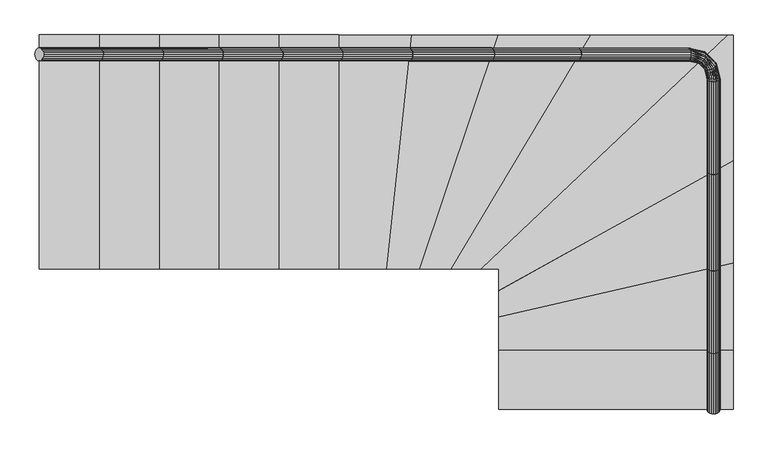
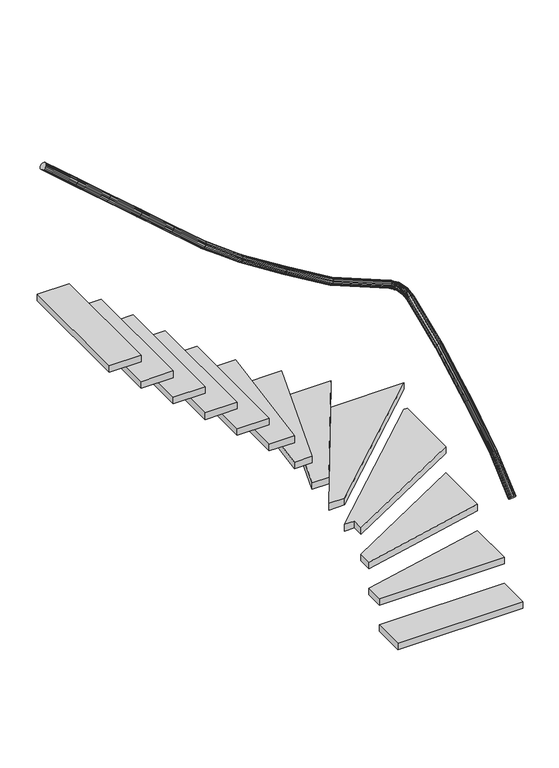
"""IFC4 building model written with IfcOpenShell, lengths in millimetres: stair geometry, 0_3d."""

import ifcopenshell
import ifcopenshell.guid

model = None  # the IFC model being written
_history = None  # IfcOwnerHistory: only IFC2X3 demands one
_inside = {}  # id of a spatial element -> (the spatial element, [elements in it])
_under = {}  # id of a project, library or spatial element -> (it, [spatial elements below it])
_declared = {}  # id of a project -> (the project, [libraries it declares])
_typed = {}  # id of a type object -> (the type object, [elements of that type])
_made_of = {}  # id of a material, layer set ... -> (it, [elements and type objects made of it])


def new_model(schema):
    """Start an empty IFC model of exactly this schema.

    Asked for "IFC4X3", IfcOpenShell would pick the latest addendum, in which some entities
    have other attributes; the version numbers below select the first issue.
    IFC2X3 requires an IfcOwnerHistory on every rooted entity: one is made here for all.
    """
    global model, _history
    if schema == "IFC4X3":
        model = ifcopenshell.file(schema_version=(4, 3, 0, 0))
    else:
        model = ifcopenshell.file(schema=schema)
    _inside.clear()
    _under.clear()
    _declared.clear()
    _typed.clear()
    _made_of.clear()
    _history = None
    if model.schema == "IFC2X3":
        org = make("IfcOrganization", Name="unknown")
        user = make(
            "IfcPersonAndOrganization",
            ThePerson=make("IfcPerson", FamilyName="unknown"),
            TheOrganization=org,
        )
        app = make(
            "IfcApplication",
            ApplicationDeveloper=org,
            Version="unknown",
            ApplicationFullName="unknown",
            ApplicationIdentifier="unknown",
        )
        _history = make(
            "IfcOwnerHistory",
            OwningUser=user,
            OwningApplication=app,
            ChangeAction="ADDED",
            CreationDate=0,
        )
    return model


def make(cls, **values):
    """One entity of the class cls with the attributes given. An attribute that is None is left unset."""
    return model.create_entity(
        cls, **{name: value for name, value in values.items() if value is not None}
    )


def rooted(cls, **values):
    """An entity with a GlobalId (a new one), such as an element, a storey or a relation."""
    return make(cls, GlobalId=ifcopenshell.guid.new(), OwnerHistory=_history, **values)


def si_unit(unit_type, name, prefix=None):
    """IfcSIUnit, for example si_unit("LENGTHUNIT", "METRE", prefix="MILLI")."""
    return make("IfcSIUnit", UnitType=unit_type, Prefix=prefix, Name=name)


def assignment(units):
    """IfcUnitAssignment: the units of a project."""
    return None if units is None else make("IfcUnitAssignment", Units=units)


def point(xyz):
    """IfcCartesianPoint."""
    return None if xyz is None else make("IfcCartesianPoint", Coordinates=xyz)


def direction(xyz):
    """IfcDirection."""
    return None if xyz is None else make("IfcDirection", DirectionRatios=xyz)


def frame(location, z_axis=None, x_axis=None):
    """IfcAxis2Placement3D, a coordinate frame: its origin and axes. An axis left out is left unset."""
    return make(
        "IfcAxis2Placement3D",
        Location=point(location),
        Axis=direction(z_axis),
        RefDirection=direction(x_axis),
    )


def origin():
    """The frame at (0, 0, 0) with its axes left unset."""
    return frame((0.0, 0.0, 0.0))


def origin_with_axes():
    """The frame at (0, 0, 0) with the z axis (0, 0, 1) and the x axis (1, 0, 0) written out."""
    return frame((0.0, 0.0, 0.0), z_axis=(0.0, 0.0, 1.0), x_axis=(1.0, 0.0, 0.0))


def place(relative_to, where):
    """IfcLocalPlacement: puts the frame where relative to a parent placement (None: the world)."""
    return make(
        "IfcLocalPlacement", PlacementRelTo=relative_to, RelativePlacement=where
    )


def context(
    kind, dimensions, precision=None, world=None, true_north=None, identifier=None
):
    """IfcGeometricRepresentationContext, for example the 3D "Model" context."""
    return make(
        "IfcGeometricRepresentationContext",
        ContextIdentifier=identifier,
        ContextType=kind,
        CoordinateSpaceDimension=dimensions,
        Precision=precision,
        WorldCoordinateSystem=world,
        TrueNorth=true_north,
    )


def project(units=None, contexts=None):
    """IfcProject with its units and contexts."""
    return rooted(
        "IfcProject",
        Name="project",
        RepresentationContexts=contexts,
        UnitsInContext=assignment(units),
    )


def spatial(cls, under=None, at=None, **own):
    """A site, building, storey or space (cls), placed at a placement, below another one or the project."""
    s = rooted(cls, ObjectPlacement=at, **own)
    if under is not None:
        _under.setdefault(under.id(), (under, []))[1].append(s)
    return s


def polyline(points):
    """IfcPolyline through the points."""
    return make("IfcPolyline", Points=[point(p) for p in points])


def outline(outer, holes=None, kind="AREA"):
    """IfcArbitraryClosedProfileDef: a profile drawn as a closed curve; with holes, ...WithVoids."""
    if holes is None:
        return make("IfcArbitraryClosedProfileDef", ProfileType=kind, OuterCurve=outer)
    return make(
        "IfcArbitraryProfileDefWithVoids",
        ProfileType=kind,
        OuterCurve=outer,
        InnerCurves=holes,
    )


def extrude(swept, where, along, depth):
    """IfcExtrudedAreaSolid: the profile swept, set in the frame where, extruded along a direction by depth."""
    return make(
        "IfcExtrudedAreaSolid",
        SweptArea=swept,
        Position=where,
        ExtrudedDirection=direction(along),
        Depth=depth,
    )


def faces_of(points, faces, orient=None, outer=None):
    """IfcFace entities. A face is a list of loops; a loop is a list of indices into points, from 0.

    orient and outer hold one flag for each loop. By default every Orientation is true, the
    first loop of a face is its IfcFaceOuterBound and the others are IfcFaceBound.
    """
    made = []
    for i, loops in enumerate(faces):
        bounds = []
        for j, loop in enumerate(loops):
            is_outer = j == 0 if outer is None else outer[i][j]
            bounds.append(
                make(
                    "IfcFaceOuterBound" if is_outer else "IfcFaceBound",
                    Bound=make("IfcPolyLoop", Polygon=[points[k] for k in loop]),
                    Orientation=True if orient is None else orient[i][j],
                )
            )
        made.append(make("IfcFace", Bounds=bounds))
    return made


def faceted_brep(points, faces, orient=None, outer=None, voids=None):
    """IfcFacetedBrep: a solid bounded by flat faces; with voids (closed shells), ...WithVoids."""
    shared = [point(p) for p in points]
    hull = make("IfcClosedShell", CfsFaces=faces_of(shared, faces, orient, outer))
    if voids is None:
        return make("IfcFacetedBrep", Outer=hull)
    return make(
        "IfcFacetedBrepWithVoids",
        Outer=hull,
        Voids=[
            make(cls, CfsFaces=faces_of(shared, fs, o, b)) for cls, fs, o, b in voids
        ],
    )


def shape(context_of_items, identifier, shape_type, items):
    """IfcShapeRepresentation: the items that make up one representation, for example the "Body"."""
    return make(
        "IfcShapeRepresentation",
        ContextOfItems=context_of_items,
        RepresentationIdentifier=identifier,
        RepresentationType=shape_type,
        Items=items,
    )


def source(mapping_origin, context_of_items, identifier, shape_type, items):
    """IfcRepresentationMap: a shape defined once, which mapped items show again and again."""
    return make(
        "IfcRepresentationMap",
        MappingOrigin=mapping_origin,
        MappedRepresentation=shape(context_of_items, identifier, shape_type, items),
    )


def transform(
    local_origin,
    x_axis=None,
    y_axis=None,
    z_axis=None,
    scale=None,
    scale2=None,
    scale3=None,
    uniform=True,
):
    """IfcCartesianTransformationOperator3D, or its non-uniform kind. x_axis, y_axis, z_axis: its Axis1, 2, 3."""
    if uniform:
        return make(
            "IfcCartesianTransformationOperator3D",
            Axis1=direction(x_axis),
            Axis2=direction(y_axis),
            LocalOrigin=point(local_origin),
            Scale=scale,
            Axis3=direction(z_axis),
        )
    return make(
        "IfcCartesianTransformationOperator3DnonUniform",
        Axis1=direction(x_axis),
        Axis2=direction(y_axis),
        LocalOrigin=point(local_origin),
        Scale=scale,
        Axis3=direction(z_axis),
        Scale2=scale2,
        Scale3=scale3,
    )


def mapped(mapping_source, mapping_target):
    """IfcMappedItem: shows the shape of a source again, moved by a transform."""
    return make(
        "IfcMappedItem", MappingSource=mapping_source, MappingTarget=mapping_target
    )


def made_of(thing, what):
    """Note that an element or type object is made of a material, layer set ...; save() writes the relation."""
    if what is not None:
        _made_of.setdefault(what.id(), (what, []))[1].append(thing)
    return thing


def element(
    cls,
    number,
    at=None,
    inside=None,
    cuts=None,
    type_object=None,
    material=None,
    context=None,
    identifier="Body",
    shape_type=None,
    held_by="IfcProductDefinitionShape",
    body=None,
    shapes=None,
    **own,
):
    """One element of the class cls, such as IfcWall. Its Tag is "e" and its number.

    at: its placement. inside: the storey or other place that contains it. cuts: it is an
    opening in that element (IfcRelVoidsElement). A single representation is given by context,
    identifier, shape_type and body (its items); several are given by shapes. held_by: the class
    of the entity that holds the representations. save() writes the other relations.
    """
    e = rooted(cls, Tag="e%d" % number, ObjectPlacement=at, **own)
    if body is not None:
        shapes = [shape(context, identifier, shape_type, body)]
    if shapes is not None:
        e.Representation = make(held_by, Representations=shapes)
    if inside is not None:
        _inside.setdefault(inside.id(), (inside, []))[1].append(e)
    if cuts is not None:
        rooted(
            "IfcRelVoidsElement", RelatingBuildingElement=cuts, RelatedOpeningElement=e
        )
    if type_object is not None:
        _typed.setdefault(type_object.id(), (type_object, []))[1].append(e)
    return made_of(e, material)


def aggregate(whole, parts):
    """IfcRelAggregates: a whole, such as a stair, and the parts it consists of."""
    return rooted("IfcRelAggregates", RelatingObject=whole, RelatedObjects=parts)


def save(model, path):
    """Write the relations noted so far, then the file.

    IfcRelAggregates (storeys below a building ...), IfcRelContainedInSpatialStructure (elements
    in a storey), IfcRelDefinesByType, IfcRelAssociatesMaterial and IfcRelDeclares: one each for
    every whole, place, type object, material and project.
    """
    for whole, parts in _under.values():
        aggregate(whole, parts)
    for where, things in _inside.values():
        rooted(
            "IfcRelContainedInSpatialStructure",
            RelatedElements=things,
            RelatingStructure=where,
        )
    for kind, things in _typed.values():
        rooted("IfcRelDefinesByType", RelatedObjects=things, RelatingType=kind)
    for what, things in _made_of.values():
        rooted("IfcRelAssociatesMaterial", RelatedObjects=things, RelatingMaterial=what)
    for by, libraries in _declared.values():
        rooted("IfcRelDeclares", RelatingContext=by, RelatedDefinitions=libraries)
    model.write(path)


def stair_d2e62eaa(model_context):
    return source(origin(), model_context, "Body", "SolidModel", [
        extrude(outline(polyline([(1597.2416565, 556.9712063), (1477.0914164, 556.9712063), (1776.8509962, 1456.9712063), (2132.6926944, 1456.9712063), (1597.2416565, 556.9712063)])), frame((0.0, 0.0, 1000.0), z_axis=(0.0, 0.0, 1.0), x_axis=(1.0, 0.0, 0.0)), (0.0, 0.0, 1.0), 50.0),
        extrude(outline(polyline([(1781.5730429, 246.9712063), (1781.5730429, 374.004016), (2681.5730429, 579.9383967), (2681.5730429, 246.9712063), (1781.5730429, 246.9712063)])), frame((0.0, 0.0, 200.0), z_axis=(0.0, 0.0, 1.0), x_axis=(1.0, 0.0, 0.0)), (0.0, 0.0, 1.0), 50.0),
        faceted_brep([(1747.6858023, 1405.7476192, 2062.7493649), (1751.8710312, 1406.9712063, 2069.5592366), (1756.0562602, 1405.7476192, 2076.3691083), (1759.8318097, 1402.1966312, 2082.5123824), (1762.8281028, 1396.6658376, 2087.3877122), (1764.7518414, 1389.6966312, 2090.5178667), (1765.4147166, 1381.9712063, 2091.5964444), (1764.7518414, 1374.2457815, 2090.5178667), (1762.8281028, 1367.276575, 2087.3877122), (1759.8318097, 1361.7457815, 2082.5123824), (1756.0562602, 1358.1947934, 2076.3691083), (1751.8710312, 1356.9712063, 2069.5592366), (1747.6858023, 1358.1947934, 2062.7493649), (1743.9102527, 1361.7457815, 2056.6060909), (1740.9139596, 1367.276575, 2051.730761), (1738.9902211, 1374.2457815, 2048.6006065), (1738.3273459, 1381.9712063, 2047.5220288), (1738.9902211, 1389.6966312, 2048.6006065), (1740.9139596, 1396.6658376, 2051.730761), (1743.9102527, 1402.1966312, 2056.6060909), (1441.2565059, 1405.7476192, 2276.1520608), (1436.7292732, 1406.9712063, 2269.5592366), (1432.2020405, 1405.7476192, 2262.9664125), (1428.1179649, 1402.1966312, 2257.0189399), (1424.8768241, 1396.6658376, 2252.2989989), (1422.7958836, 1389.6966312, 2249.2686103), (1422.0788404, 1381.9712063, 2248.2244095), (1422.7958836, 1374.2457815, 2249.2686103), (1424.8768241, 1367.276575, 2252.2989989), (1428.1179649, 1361.7457815, 2257.0189399), (1432.2020405, 1358.1947934, 2262.9664125), (1436.7292732, 1356.9712063, 2269.5592366), (1441.2565059, 1358.1947934, 2276.1520608), (1445.3405815, 1361.7457815, 2282.0995333), (1448.5817223, 1367.276575, 2286.8194743), (1450.6626628, 1374.2457815, 2289.8498629), (1451.379706, 1381.9712063, 2290.8940637), (1450.6626628, 1389.6966312, 2289.8498629), (1448.5817223, 1396.6658376, 2286.8194743), (1445.3405815, 1402.1966312, 2282.0995333)], [[[0, 1, 2, 3, 4, 5, 6, 7, 8, 9, 10, 11, 12, 13, 14, 15, 16, 17, 18, 19]], [[20, 21, 22, 23, 24, 25, 26, 27, 28, 29, 30, 31, 32, 33, 34, 35, 36, 37, 38, 39]], [[2, 1, 21, 20]], [[3, 2, 20, 39]], [[4, 3, 39, 38]], [[5, 4, 38, 37]], [[6, 5, 37, 36]], [[7, 6, 36, 35]], [[8, 7, 35, 34]], [[9, 8, 34, 33]], [[10, 9, 33, 32]], [[11, 10, 32, 31]], [[12, 11, 31, 30]], [[13, 12, 30, 29]], [[14, 13, 29, 28]], [[15, 14, 28, 27]], [[16, 15, 27, 26]], [[17, 16, 26, 25]], [[18, 17, 25, 24]], [[19, 18, 24, 23]], [[0, 19, 23, 22]], [[1, 0, 22, 21]]]),
        extrude(outline(polyline([(1711.5730429, 556.9712063), (1597.2416565, 556.9712063), (2132.6926944, 1456.9712063), (2658.9026268, 1456.9712063), (1711.5730429, 556.9712063)])), frame((0.0, 0.0, 800.0), z_axis=(0.0, 0.0, 1.0), x_axis=(1.0, 0.0, 0.0)), (0.0, 0.0, 1.0), 50.0),
        extrude(outline(polyline([(476.9712063, 556.9712063), (246.9712063, 556.9712063), (246.9712063, 1456.9712063), (476.9712063, 1456.9712063), (476.9712063, 556.9712063)])), frame((0.0, 0.0, 2200.0), z_axis=(0.0, 0.0, 1.0), x_axis=(1.0, 0.0, 0.0)), (0.0, 0.0, 1.0), 50.0),
        faceted_brep([(2630.3494558, 1289.6562562, 1611.0200809), (2631.5730429, 1286.5654708, 1618.3905793), (2630.3494558, 1283.4746854, 1625.7610778), (2626.7984678, 1280.6864477, 1632.4101004), (2621.2676742, 1278.4736897, 1637.6867947), (2614.2984678, 1277.0530116, 1641.074641), (2606.5730429, 1276.5634793, 1642.2420132), (2598.8476181, 1277.0530116, 1641.074641), (2591.8784116, 1278.4736897, 1637.6867947), (2586.3476181, 1280.6864477, 1632.4101004), (2582.79663, 1283.4746854, 1625.7610778), (2581.5730429, 1286.5654708, 1618.3905793), (2582.79663, 1289.6562562, 1611.0200809), (2586.3476181, 1292.4444939, 1604.3710583), (2591.8784116, 1294.6572519, 1599.094364), (2598.8476181, 1296.07793, 1595.7065177), (2606.5730429, 1296.5674623, 1594.5391455), (2614.2984678, 1296.07793, 1595.7065177), (2621.2676742, 1294.6572519, 1599.094364), (2626.7984678, 1292.4444939, 1604.3710583), (2616.5930378, 1348.981721, 1644.4666407), (2617.4087642, 1344.9399789, 1651.4217307), (2615.9975628, 1340.119684, 1657.6960081), (2612.4975719, 1334.9926804, 1662.6753028), (2607.2513949, 1330.060835, 1665.8722068), (2600.7725643, 1325.8069111, 1666.9737849), (2593.6952731, 1322.6473125, 1665.8722068), (2586.7122958, 1320.8913226, 1662.6753028), (2580.507175, 1320.71083, 1657.6960081), (2575.6873111, 1322.1235026, 1651.4217307), (2572.7245059, 1324.9910581, 1644.4666407), (2571.9087795, 1329.0328002, 1637.5115507), (2573.3199809, 1333.8530951, 1631.2372733), (2576.8199719, 1338.9800987, 1626.2579786), (2582.0661488, 1343.9119441, 1623.0610746), (2588.5449795, 1348.165868, 1621.9594966), (2595.6222707, 1351.3254666, 1623.0610746), (2602.605248, 1353.0814565, 1626.2579786), (2608.8103688, 1353.2619491, 1631.2372733), (2613.6302327, 1351.8492765, 1637.5115507), (2573.4194125, 1392.0411015, 1672.0001373), (2576.2683384, 1389.0986856, 1678.9715199), (2577.6691227, 1384.2945329, 1685.260495), (2577.4846471, 1378.0989073, 1690.251454), (2575.7329691, 1371.11828, 1693.4558469), (2572.5855554, 1364.0359633, 1694.5600054), (2568.3504965, 1357.5452238, 1693.4558469), (2563.4423498, 1352.2814202, 1690.251454), (2558.3415586, 1348.7598103, 1685.260495), (2553.547424, 1347.3251138, 1678.9715199), (2549.5292294, 1348.1177689, 1672.0001373), (2546.6803035, 1351.0601849, 1665.0287546), (2545.2795191, 1355.8643376, 1658.7397795), (2545.4639948, 1362.0599631, 1653.7488206), (2547.2156727, 1369.0405904, 1650.5444277), (2550.3630865, 1376.1229071, 1649.4402691), (2554.5981453, 1382.6136466, 1650.5444277), (2559.5062921, 1387.8774503, 1653.7488206), (2564.6070832, 1391.3990601, 1658.7397795), (2569.4012178, 1392.8337566, 1665.0287546), (2510.8572333, 1406.9712063, 1697.6556493), (2513.867569, 1405.7476192, 1705.05937), (2516.583232, 1402.1966312, 1711.7383629), (2518.7383944, 1396.6658376, 1717.0388417), (2520.1220939, 1389.6966312, 1720.4419586), (2520.5988842, 1381.9712063, 1721.6145928), (2520.1220939, 1374.2457815, 1720.4419586), (2518.7383944, 1367.276575, 1717.0388417), (2516.583232, 1361.7457815, 1711.7383629), (2513.867569, 1358.1947934, 1705.05937), (2510.8572333, 1356.9712063, 1697.6556493), (2507.8468977, 1358.1947934, 1690.2519286), (2505.1312346, 1361.7457815, 1683.5729357), (2502.9760722, 1367.276575, 1678.2724569), (2501.5923728, 1374.2457815, 1674.86934), (2501.1155825, 1381.9712063, 1673.6967059), (2501.5923728, 1389.6966312, 1674.86934), (2502.9760722, 1396.6658376, 1678.2724569), (2505.1312346, 1402.1966312, 1683.5729357), (2507.8468977, 1405.7476192, 1690.2519286), (2091.6401721, 1405.7476192, 1876.7360506), (2088.0717746, 1406.9712063, 1869.5592366), (2084.503377, 1405.7476192, 1862.3824226), (2081.2842791, 1402.1966312, 1855.9081251), (2078.7295885, 1396.6658376, 1850.7700936), (2077.0893762, 1389.6966312, 1847.4712742), (2076.5241975, 1381.9712063, 1846.3345786), (2077.0893762, 1374.2457815, 1847.4712742), (2078.7295885, 1367.276575, 1850.7700936), (2081.2842791, 1361.7457815, 1855.9081251), (2084.503377, 1358.1947934, 1862.3824226), (2088.0717746, 1356.9712063, 1869.5592366), (2091.6401721, 1358.1947934, 1876.7360506), (2094.8592701, 1361.7457815, 1883.2103481), (2097.4139607, 1367.276575, 1888.3483797), (2099.054173, 1374.2457815, 1891.647199), (2099.6193516, 1381.9712063, 1892.7838947), (2099.054173, 1389.6966312, 1891.647199), (2097.4139607, 1396.6658376, 1888.3483797), (2094.8592701, 1402.1966312, 1883.2103481)], [[[0, 1, 2, 3, 4, 5, 6, 7, 8, 9, 10, 11, 12, 13, 14, 15, 16, 17, 18, 19]], [[2, 1, 20]], [[21, 2, 20]], [[3, 2, 21]], [[22, 3, 21]], [[4, 3, 22]], [[23, 4, 22]], [[5, 4, 23]], [[24, 5, 23]], [[6, 5, 24]], [[25, 6, 24]], [[7, 6, 25]], [[26, 7, 25]], [[8, 7, 26]], [[27, 8, 26]], [[9, 8, 27]], [[28, 9, 27]], [[10, 9, 28]], [[29, 10, 28]], [[11, 10, 29]], [[30, 11, 29]], [[12, 11, 30]], [[31, 12, 30]], [[13, 12, 31]], [[32, 13, 31]], [[14, 13, 32]], [[33, 14, 32]], [[15, 14, 33]], [[34, 15, 33]], [[16, 15, 34]], [[35, 16, 34]], [[17, 16, 35]], [[36, 17, 35]], [[18, 17, 36]], [[37, 18, 36]], [[19, 18, 37]], [[38, 19, 37]], [[0, 19, 38]], [[39, 0, 38]], [[1, 0, 39]], [[20, 1, 39]], [[21, 20, 40]], [[41, 21, 40]], [[22, 21, 41]], [[42, 22, 41]], [[23, 22, 42]], [[43, 23, 42]], [[24, 23, 43]], [[44, 24, 43]], [[25, 24, 44]], [[45, 25, 44]], [[26, 25, 45]], [[46, 26, 45]], [[27, 26, 46]], [[47, 27, 46]], [[28, 27, 47]], [[48, 28, 47]], [[29, 28, 48]], [[49, 29, 48]], [[30, 29, 49]], [[50, 30, 49]], [[31, 30, 50]], [[51, 31, 50]], [[32, 31, 51]], [[52, 32, 51]], [[33, 32, 52]], [[53, 33, 52]], [[34, 33, 53]], [[54, 34, 53]], [[35, 34, 54]], [[55, 35, 54]], [[36, 35, 55]], [[56, 36, 55]], [[37, 36, 56]], [[57, 37, 56]], [[38, 37, 57]], [[58, 38, 57]], [[39, 38, 58]], [[59, 39, 58]], [[20, 39, 59]], [[40, 20, 59]], [[41, 40, 60]], [[61, 41, 60]], [[42, 41, 61]], [[62, 42, 61]], [[43, 42, 62]], [[63, 43, 62]], [[44, 43, 63]], [[64, 44, 63]], [[45, 44, 64]], [[65, 45, 64]], [[46, 45, 65]], [[66, 46, 65]], [[47, 46, 66]], [[67, 47, 66]], [[48, 47, 67]], [[68, 48, 67]], [[49, 48, 68]], [[69, 49, 68]], [[50, 49, 69]], [[70, 50, 69]], [[51, 50, 70]], [[71, 51, 70]], [[52, 51, 71]], [[72, 52, 71]], [[53, 52, 72]], [[73, 53, 72]], [[54, 53, 73]], [[74, 54, 73]], [[55, 54, 74]], [[75, 55, 74]], [[56, 55, 75]], [[76, 56, 75]], [[57, 56, 76]], [[77, 57, 76]], [[58, 57, 77]], [[78, 58, 77]], [[59, 58, 78]], [[79, 59, 78]], [[40, 59, 79]], [[60, 40, 79]], [[80, 81, 82, 83, 84, 85, 86, 87, 88, 89, 90, 91, 92, 93, 94, 95, 96, 97, 98, 99]], [[61, 60, 81, 80]], [[62, 61, 80, 99]], [[63, 62, 99, 98]], [[64, 63, 98, 97]], [[65, 64, 97, 96]], [[66, 65, 96, 95]], [[67, 66, 95, 94]], [[68, 67, 94, 93]], [[69, 68, 93, 92]], [[70, 69, 92, 91]], [[71, 70, 91, 90]], [[72, 71, 90, 89]], [[73, 72, 89, 88]], [[74, 73, 88, 87]], [[75, 74, 87, 86]], [[76, 75, 86, 85]], [[77, 76, 85, 84]], [[78, 77, 84, 83]], [[79, 78, 83, 82]], [[60, 79, 82, 81]]]),
        faceted_brep([(2630.3494558, 935.1107738, 1462.3430272), (2631.5730429, 931.6520604, 1469.5592366), (2630.3494558, 928.193347, 1476.775446), (2626.7984678, 925.0731965, 1483.2852826), (2621.2676742, 922.5970311, 1488.4515182), (2614.2984678, 921.0072351, 1491.7684456), (2606.5730429, 920.4594287, 1492.9113809), (2598.8476181, 921.0072351, 1491.7684456), (2591.8784116, 922.5970311, 1488.4515182), (2586.3476181, 925.0731965, 1483.2852826), (2582.79663, 928.193347, 1476.775446), (2581.5730429, 931.6520604, 1469.5592366), (2582.79663, 935.1107738, 1462.3430272), (2586.3476181, 938.2309242, 1455.8331906), (2591.8784116, 940.7070896, 1450.666955), (2598.8476181, 942.2968856, 1447.3500276), (2606.5730429, 942.844692, 1446.2070923), (2614.2984678, 942.2968856, 1447.3500276), (2621.2676742, 940.7070896, 1450.666955), (2626.7984678, 938.2309242, 1455.8331906), (2630.3494558, 1283.4746854, 1625.7610778), (2631.5730429, 1286.5654708, 1618.3905793), (2630.3494558, 1289.6562562, 1611.0200809), (2626.7984678, 1292.4444939, 1604.3710583), (2621.2676742, 1294.6572519, 1599.094364), (2614.2984678, 1296.07793, 1595.7065177), (2606.5730429, 1296.5674623, 1594.5391455), (2598.8476181, 1296.07793, 1595.7065177), (2591.8784116, 1294.6572519, 1599.094364), (2586.3476181, 1292.4444939, 1604.3710583), (2582.79663, 1289.6562562, 1611.0200809), (2581.5730429, 1286.5654708, 1618.3905793), (2582.79663, 1283.4746854, 1625.7610778), (2586.3476181, 1280.6864477, 1632.4101004), (2591.8784116, 1278.4736897, 1637.6867947), (2598.8476181, 1277.0530116, 1641.074641), (2606.5730429, 1276.5634793, 1642.2420132), (2614.2984678, 1277.0530116, 1641.074641), (2621.2676742, 1278.4736897, 1637.6867947), (2626.7984678, 1280.6864477, 1632.4101004)], [[[0, 1, 2, 3, 4, 5, 6, 7, 8, 9, 10, 11, 12, 13, 14, 15, 16, 17, 18, 19]], [[20, 21, 22, 23, 24, 25, 26, 27, 28, 29, 30, 31, 32, 33, 34, 35, 36, 37, 38, 39]], [[2, 1, 21, 20]], [[3, 2, 20, 39]], [[4, 3, 39, 38]], [[5, 4, 38, 37]], [[6, 5, 37, 36]], [[7, 6, 36, 35]], [[8, 7, 35, 34]], [[9, 8, 34, 33]], [[10, 9, 33, 32]], [[11, 10, 32, 31]], [[12, 11, 31, 30]], [[13, 12, 30, 29]], [[14, 13, 29, 28]], [[15, 14, 28, 27]], [[16, 15, 27, 26]], [[17, 16, 26, 25]], [[18, 17, 25, 24]], [[19, 18, 24, 23]], [[0, 19, 23, 22]], [[1, 0, 22, 21]]]),
        faceted_brep([(1161.9614386, 1405.7476192, 2463.3241664), (1166.9712063, 1406.9712063, 2469.5592366), (1171.980974, 1405.7476192, 2475.7943068), (1176.5003508, 1402.1966312, 2481.419045), (1180.0869485, 1396.6658376, 2485.8828624), (1182.3896859, 1389.6966312, 2488.7488096), (1183.1831552, 1381.9712063, 2489.7363478), (1182.3896859, 1374.2457815, 2488.7488096), (1180.0869485, 1367.276575, 2485.8828624), (1176.5003508, 1361.7457815, 2481.419045), (1171.980974, 1358.1947934, 2475.7943068), (1166.9712063, 1356.9712063, 2469.5592366), (1161.9614386, 1358.1947934, 2463.3241664), (1157.4420619, 1361.7457815, 2457.6994282), (1153.8554642, 1367.276575, 2453.2356108), (1151.5527267, 1374.2457815, 2450.3696636), (1150.7592575, 1381.9712063, 2449.3821255), (1151.5527267, 1389.6966312, 2450.3696636), (1153.8554642, 1396.6658376, 2453.2356108), (1157.4420619, 1402.1966312, 2457.6994282), (942.2155975, 1405.7476192, 2675.5902865), (936.9712063, 1406.9712063, 2669.5592366), (931.7268152, 1405.7476192, 2663.5281868), (926.9957815, 1402.1966312, 2658.0874981), (923.241212, 1396.6658376, 2653.7697431), (920.83063, 1389.6966312, 2650.9975738), (920.0, 1381.9712063, 2650.0423493), (920.83063, 1374.2457815, 2650.9975738), (923.241212, 1367.276575, 2653.7697431), (926.9957815, 1361.7457815, 2658.0874981), (931.7268152, 1358.1947934, 2663.5281868), (936.9712063, 1356.9712063, 2669.5592366), (942.2155975, 1358.1947934, 2675.5902865), (946.9466311, 1361.7457815, 2681.0309751), (950.7012007, 1367.276575, 2685.3487301), (953.1117827, 1374.2457815, 2688.1208994), (953.9424127, 1381.9712063, 2689.0761239), (953.1117827, 1389.6966312, 2688.1208994), (950.7012007, 1396.6658376, 2685.3487301), (946.9466311, 1402.1966312, 2681.0309751)], [[[0, 1, 2, 3, 4, 5, 6, 7, 8, 9, 10, 11, 12, 13, 14, 15, 16, 17, 18, 19]], [[20, 21, 22, 23, 24, 25, 26, 27, 28, 29, 30, 31, 32, 33, 34, 35, 36, 37, 38, 39]], [[2, 1, 21, 20]], [[3, 2, 20, 39]], [[4, 3, 39, 38]], [[5, 4, 38, 37]], [[6, 5, 37, 36]], [[7, 6, 36, 35]], [[8, 7, 35, 34]], [[9, 8, 34, 33]], [[10, 9, 33, 32]], [[11, 10, 32, 31]], [[12, 11, 31, 30]], [[13, 12, 30, 29]], [[14, 13, 29, 28]], [[15, 14, 28, 27]], [[16, 15, 27, 26]], [[17, 16, 26, 25]], [[18, 17, 25, 24]], [[19, 18, 24, 23]], [[0, 19, 23, 22]], [[1, 0, 22, 21]]]),
        extrude(outline(polyline([(1.2235871, -7.9923213), (0.0, 0.0), (1.2235871, 7.9923214), (4.7745751, 15.2022986), (10.3053687, 20.9241691), (17.2745751, 24.5978359), (25.0, 25.8636953), (32.7254248, 24.5978359), (39.6946313, 20.9241691), (45.2254248, 15.2022986), (48.7764129, 7.9923214), (50.0, 0.0), (48.7764129, -7.9923213), (45.2254248, -15.2022986), (39.6946313, -20.924169), (32.7254248, -24.5978359), (25.0, -25.8636953), (17.2745751, -24.5978359), (10.3053687, -20.924169), (4.7745751, -15.2022986), (1.2235871, -7.9923213)])), frame((476.9712063, 1406.9712063, 3069.5592366), z_axis=(-0.7546055221634675, 0.0, 0.6561787149248295), x_axis=(0.0, -1.0, 0.0)), (0.0, 0.0, 1.0), 304.7950131),
        extrude(outline(polyline([(936.9712063, 556.9712063), (706.9712063, 556.9712063), (706.9712063, 1456.9712063), (936.9712063, 1456.9712063), (936.9712063, 556.9712063)])), frame((0.0, 0.0, 1800.0), z_axis=(0.0, 0.0, 1.0), x_axis=(1.0, 0.0, 0.0)), (0.0, 0.0, 1.0), 50.0),
        faceted_brep([(2630.3494558, 566.8246344, 1262.6622263), (2631.5730429, 562.7771983, 1269.5592366), (2630.3494558, 558.7297622, 1276.4562469), (2626.7984678, 555.0785174, 1282.6781298), (2621.2676742, 552.180873, 1287.615844), (2614.2984678, 550.3204709, 1290.7860517), (2606.5730429, 549.67942, 1291.8784308), (2598.8476181, 550.3204709, 1290.7860517), (2591.8784116, 552.180873, 1287.615844), (2586.3476181, 555.0785174, 1282.6781298), (2582.79663, 558.7297622, 1276.4562469), (2581.5730429, 562.7771983, 1269.5592366), (2582.79663, 566.8246344, 1262.6622263), (2586.3476181, 570.4758792, 1256.4403434), (2591.8784116, 573.3735235, 1251.5026292), (2598.8476181, 575.2339257, 1248.3324215), (2606.5730429, 575.8749766, 1247.2400424), (2614.2984678, 575.2339257, 1248.3324215), (2621.2676742, 573.3735235, 1251.5026292), (2626.7984678, 570.4758792, 1256.4403434), (2630.3494558, 928.193347, 1476.775446), (2631.5730429, 931.6520604, 1469.5592366), (2630.3494558, 935.1107738, 1462.3430272), (2626.7984678, 938.2309242, 1455.8331906), (2621.2676742, 940.7070896, 1450.666955), (2614.2984678, 942.2968856, 1447.3500276), (2606.5730429, 942.844692, 1446.2070923), (2598.8476181, 942.2968856, 1447.3500276), (2591.8784116, 940.7070896, 1450.666955), (2586.3476181, 938.2309242, 1455.8331906), (2582.79663, 935.1107738, 1462.3430272), (2581.5730429, 931.6520604, 1469.5592366), (2582.79663, 928.193347, 1476.775446), (2586.3476181, 925.0731965, 1483.2852826), (2591.8784116, 922.5970311, 1488.4515182), (2598.8476181, 921.0072351, 1491.7684456), (2606.5730429, 920.4594287, 1492.9113809), (2614.2984678, 921.0072351, 1491.7684456), (2621.2676742, 922.5970311, 1488.4515182), (2626.7984678, 925.0731965, 1483.2852826)], [[[0, 1, 2, 3, 4, 5, 6, 7, 8, 9, 10, 11, 12, 13, 14, 15, 16, 17, 18, 19]], [[20, 21, 22, 23, 24, 25, 26, 27, 28, 29, 30, 31, 32, 33, 34, 35, 36, 37, 38, 39]], [[2, 1, 21, 20]], [[3, 2, 20, 39]], [[4, 3, 39, 38]], [[5, 4, 38, 37]], [[6, 5, 37, 36]], [[7, 6, 36, 35]], [[8, 7, 35, 34]], [[9, 8, 34, 33]], [[10, 9, 33, 32]], [[11, 10, 32, 31]], [[12, 11, 31, 30]], [[13, 12, 30, 29]], [[14, 13, 29, 28]], [[15, 14, 28, 27]], [[16, 15, 27, 26]], [[17, 16, 26, 25]], [[18, 17, 25, 24]], [[19, 18, 24, 23]], [[0, 19, 23, 22]], [[1, 0, 22, 21]]]),
        extrude(outline(polyline([(1.2235871, -7.9923213), (0.0, 0.0), (1.2235871, 7.9923214), (4.7745751, 15.2022986), (10.3053687, 20.9241691), (17.2745751, 24.5978359), (25.0, 25.8636953), (32.7254248, 24.5978359), (39.6946313, 20.9241691), (45.2254248, 15.2022986), (48.7764129, 7.9923214), (50.0, 0.0), (48.7764129, -7.9923213), (45.2254248, -15.2022986), (39.6946313, -20.924169), (32.7254248, -24.5978359), (25.0, -25.8636953), (17.2745751, -24.5978359), (10.3053687, -20.924169), (4.7745751, -15.2022986), (1.2235871, -7.9923213)])), frame((246.9712063, 1406.9712063, 3269.5592366), z_axis=(-0.7546055221635026, 0.0, 0.6561787149247892), x_axis=(0.0, -1.0, 0.0)), (0.0, 0.0, 1.0), 304.7950131),
        extrude(outline(polyline([(1349.2615261, 556.9712063), (1166.9712063, 556.9712063), (1166.9712063, 1456.9712063), (1444.6808866, 1456.9712063), (1349.2615261, 556.9712063)])), frame((0.0, 0.0, 1400.0), z_axis=(0.0, 0.0, 1.0), x_axis=(1.0, 0.0, 0.0)), (0.0, 0.0, 1.0), 50.0),
        extrude(outline(polyline([(1781.5730429, 16.9712063), (1781.5730429, 246.9712063), (2681.5730429, 246.9712063), (2681.5730429, 16.9712063), (1781.5730429, 16.9712063)])), origin_with_axes(), (0.0, 0.0, 1.0), 50.0),
        extrude(outline(polyline([(1.2235871, -7.9923213), (0.0, 0.0), (1.2235871, 7.9923214), (4.7745751, 15.2022986), (10.3053687, 20.9241691), (17.2745751, 24.5978359), (25.0, 25.8636953), (32.7254248, 24.5978359), (39.6946313, 20.9241691), (45.2254248, 15.2022986), (48.7764129, 7.9923214), (50.0, 0.0), (48.7764129, -7.9923213), (45.2254248, -15.2022986), (39.6946313, -20.924169), (32.7254248, -24.5978359), (25.0, -25.8636953), (17.2745751, -24.5978359), (10.3053687, -20.924169), (4.7745751, -15.2022986), (1.2235871, -7.9923213)])), frame((936.9712063, 1406.9712063, 2669.5592366), z_axis=(-0.7546055221634769, 0.0, 0.6561787149248187), x_axis=(0.0, -1.0, 0.0)), (0.0, 0.0, 1.0), 304.7950131),
        faceted_brep([(2084.503377, 1405.7476192, 1862.3824226), (2088.0717746, 1406.9712063, 1869.5592366), (2091.6401721, 1405.7476192, 1876.7360506), (2094.8592701, 1402.1966312, 1883.2103481), (2097.4139607, 1396.6658376, 1888.3483797), (2099.054173, 1389.6966312, 1891.647199), (2099.6193516, 1381.9712063, 1892.7838947), (2099.054173, 1374.2457815, 1891.647199), (2097.4139607, 1367.276575, 1888.3483797), (2094.8592701, 1361.7457815, 1883.2103481), (2091.6401721, 1358.1947934, 1876.7360506), (2088.0717746, 1356.9712063, 1869.5592366), (2084.503377, 1358.1947934, 1862.3824226), (2081.2842791, 1361.7457815, 1855.9081251), (2078.7295885, 1367.276575, 1850.7700936), (2077.0893762, 1374.2457815, 1847.4712742), (2076.5241975, 1381.9712063, 1846.3345786), (2077.0893762, 1389.6966312, 1847.4712742), (2078.7295885, 1396.6658376, 1850.7700936), (2081.2842791, 1402.1966312, 1855.9081251), (1756.0562602, 1405.7476192, 2076.3691083), (1751.8710312, 1406.9712063, 2069.5592366), (1747.6858023, 1405.7476192, 2062.7493649), (1743.9102527, 1402.1966312, 2056.6060909), (1740.9139596, 1396.6658376, 2051.730761), (1738.9902211, 1389.6966312, 2048.6006065), (1738.3273459, 1381.9712063, 2047.5220288), (1738.9902211, 1374.2457815, 2048.6006065), (1740.9139596, 1367.276575, 2051.730761), (1743.9102527, 1361.7457815, 2056.6060909), (1747.6858023, 1358.1947934, 2062.7493649), (1751.8710312, 1356.9712063, 2069.5592366), (1756.0562602, 1358.1947934, 2076.3691083), (1759.8318097, 1361.7457815, 2082.5123824), (1762.8281028, 1367.276575, 2087.3877122), (1764.7518414, 1374.2457815, 2090.5178667), (1765.4147166, 1381.9712063, 2091.5964444), (1764.7518414, 1389.6966312, 2090.5178667), (1762.8281028, 1396.6658376, 2087.3877122), (1759.8318097, 1402.1966312, 2082.5123824)], [[[0, 1, 2, 3, 4, 5, 6, 7, 8, 9, 10, 11, 12, 13, 14, 15, 16, 17, 18, 19]], [[20, 21, 22, 23, 24, 25, 26, 27, 28, 29, 30, 31, 32, 33, 34, 35, 36, 37, 38, 39]], [[2, 1, 21, 20]], [[3, 2, 20, 39]], [[4, 3, 39, 38]], [[5, 4, 38, 37]], [[6, 5, 37, 36]], [[7, 6, 36, 35]], [[8, 7, 35, 34]], [[9, 8, 34, 33]], [[10, 9, 33, 32]], [[11, 10, 32, 31]], [[12, 11, 31, 30]], [[13, 12, 30, 29]], [[14, 13, 29, 28]], [[15, 14, 28, 27]], [[16, 15, 27, 26]], [[17, 16, 26, 25]], [[18, 17, 25, 24]], [[19, 18, 24, 23]], [[0, 19, 23, 22]], [[1, 0, 22, 21]]]),
        faceted_brep([(2630.3494558, 251.7587861, 1063.1309594), (2631.5730429, 246.9712063, 1069.5592366), (2630.3494558, 242.1836266, 1075.9875138), (2626.7984678, 237.8646885, 1081.7865464), (2621.2676742, 234.4371599, 1086.3886848), (2614.2984678, 232.236551, 1089.3434395), (2606.5730429, 231.4782729, 1090.3615786), (2598.8476181, 232.236551, 1089.3434395), (2591.8784116, 234.4371599, 1086.3886848), (2586.3476181, 237.8646885, 1081.7865464), (2582.79663, 242.1836266, 1075.9875138), (2581.5730429, 246.9712063, 1069.5592366), (2582.79663, 251.7587861, 1063.1309594), (2586.3476181, 256.0777241, 1057.3319268), (2591.8784116, 259.5052528, 1052.7297884), (2598.8476181, 261.7058616, 1049.7750337), (2606.5730429, 262.4641398, 1048.7568947), (2614.2984678, 261.7058616, 1049.7750337), (2621.2676742, 259.5052528, 1052.7297884), (2626.7984678, 256.0777241, 1057.3319268), (2630.3494558, 558.7297622, 1276.4562469), (2631.5730429, 562.7771983, 1269.5592366), (2630.3494558, 566.8246344, 1262.6622263), (2626.7984678, 570.4758792, 1256.4403434), (2621.2676742, 573.3735235, 1251.5026292), (2614.2984678, 575.2339257, 1248.3324215), (2606.5730429, 575.8749766, 1247.2400424), (2598.8476181, 575.2339257, 1248.3324215), (2591.8784116, 573.3735235, 1251.5026292), (2586.3476181, 570.4758792, 1256.4403434), (2582.79663, 566.8246344, 1262.6622263), (2581.5730429, 562.7771983, 1269.5592366), (2582.79663, 558.7297622, 1276.4562469), (2586.3476181, 555.0785174, 1282.6781298), (2591.8784116, 552.180873, 1287.615844), (2598.8476181, 550.3204709, 1290.7860517), (2606.5730429, 549.67942, 1291.8784308), (2614.2984678, 550.3204709, 1290.7860517), (2621.2676742, 552.180873, 1287.615844), (2626.7984678, 555.0785174, 1282.6781298)], [[[0, 1, 2, 3, 4, 5, 6, 7, 8, 9, 10, 11, 12, 13, 14, 15, 16, 17, 18, 19]], [[20, 21, 22, 23, 24, 25, 26, 27, 28, 29, 30, 31, 32, 33, 34, 35, 36, 37, 38, 39]], [[2, 1, 21, 20]], [[3, 2, 20, 39]], [[4, 3, 39, 38]], [[5, 4, 38, 37]], [[6, 5, 37, 36]], [[7, 6, 36, 35]], [[8, 7, 35, 34]], [[9, 8, 34, 33]], [[10, 9, 33, 32]], [[11, 10, 32, 31]], [[12, 11, 31, 30]], [[13, 12, 30, 29]], [[14, 13, 29, 28]], [[15, 14, 28, 27]], [[16, 15, 27, 26]], [[17, 16, 26, 25]], [[18, 17, 25, 24]], [[19, 18, 24, 23]], [[0, 19, 23, 22]], [[1, 0, 22, 21]]]),
        extrude(outline(polyline([(246.9712063, 556.9712063), (16.9712063, 556.9712063), (16.9712063, 1456.9712063), (246.9712063, 1456.9712063), (246.9712063, 556.9712063)])), frame((0.0, 0.0, 2400.0), z_axis=(0.0, 0.0, 1.0), x_axis=(1.0, 0.0, 0.0)), (0.0, 0.0, 1.0), 50.0),
        faceted_brep([(1432.2020405, 1405.7476192, 2262.9664125), (1436.7292732, 1406.9712063, 2269.5592366), (1441.2565059, 1405.7476192, 2276.1520608), (1445.3405815, 1402.1966312, 2282.0995333), (1448.5817223, 1396.6658376, 2286.8194743), (1450.6626628, 1389.6966312, 2289.8498629), (1451.379706, 1381.9712063, 2290.8940637), (1450.6626628, 1374.2457815, 2289.8498629), (1448.5817223, 1367.276575, 2286.8194743), (1445.3405815, 1361.7457815, 2282.0995333), (1441.2565059, 1358.1947934, 2276.1520608), (1436.7292732, 1356.9712063, 2269.5592366), (1432.2020405, 1358.1947934, 2262.9664125), (1428.1179649, 1361.7457815, 2257.0189399), (1424.8768241, 1367.276575, 2252.2989989), (1422.7958836, 1374.2457815, 2249.2686103), (1422.0788404, 1381.9712063, 2248.2244095), (1422.7958836, 1389.6966312, 2249.2686103), (1424.8768241, 1396.6658376, 2252.2989989), (1428.1179649, 1402.1966312, 2257.0189399), (1171.980974, 1405.7476192, 2475.7943068), (1166.9712063, 1406.9712063, 2469.5592366), (1161.9614386, 1405.7476192, 2463.3241664), (1157.4420619, 1402.1966312, 2457.6994282), (1153.8554642, 1396.6658376, 2453.2356108), (1151.5527267, 1389.6966312, 2450.3696636), (1150.7592575, 1381.9712063, 2449.3821255), (1151.5527267, 1374.2457815, 2450.3696636), (1153.8554642, 1367.276575, 2453.2356108), (1157.4420619, 1361.7457815, 2457.6994282), (1161.9614386, 1358.1947934, 2463.3241664), (1166.9712063, 1356.9712063, 2469.5592366), (1171.980974, 1358.1947934, 2475.7943068), (1176.5003508, 1361.7457815, 2481.419045), (1180.0869485, 1367.276575, 2485.8828624), (1182.3896859, 1374.2457815, 2488.7488096), (1183.1831552, 1381.9712063, 2489.7363478), (1182.3896859, 1389.6966312, 2488.7488096), (1180.0869485, 1396.6658376, 2485.8828624), (1176.5003508, 1402.1966312, 2481.419045)], [[[0, 1, 2, 3, 4, 5, 6, 7, 8, 9, 10, 11, 12, 13, 14, 15, 16, 17, 18, 19]], [[20, 21, 22, 23, 24, 25, 26, 27, 28, 29, 30, 31, 32, 33, 34, 35, 36, 37, 38, 39]], [[2, 1, 21, 20]], [[3, 2, 20, 39]], [[4, 3, 39, 38]], [[5, 4, 38, 37]], [[6, 5, 37, 36]], [[7, 6, 36, 35]], [[8, 7, 35, 34]], [[9, 8, 34, 33]], [[10, 9, 33, 32]], [[11, 10, 32, 31]], [[12, 11, 31, 30]], [[13, 12, 30, 29]], [[14, 13, 29, 28]], [[15, 14, 28, 27]], [[16, 15, 27, 26]], [[17, 16, 26, 25]], [[18, 17, 25, 24]], [[19, 18, 24, 23]], [[0, 19, 23, 22]], [[1, 0, 22, 21]]]),
        faceted_brep([(2630.3494558, 22.2155975, 863.5281868), (2631.5730429, 16.9712063, 869.5592366), (2630.3494558, 11.7268152, 875.5902865), (2626.7984678, 6.9957815, 881.0309751), (2621.2676742, 3.241212, 885.3487301), (2614.2984678, 0.83063, 888.1208994), (2606.5730429, 0.0, 889.0761239), (2598.8476181, 0.83063, 888.1208994), (2591.8784116, 3.241212, 885.3487301), (2586.3476181, 6.9957815, 881.0309751), (2582.79663, 11.7268152, 875.5902865), (2581.5730429, 16.9712063, 869.5592366), (2582.79663, 22.2155975, 863.5281868), (2586.3476181, 26.9466311, 858.0874981), (2591.8784116, 30.7012007, 853.7697431), (2598.8476181, 33.1117827, 850.9975738), (2606.5730429, 33.9424127, 850.0423493), (2614.2984678, 33.1117827, 850.9975738), (2621.2676742, 30.7012007, 853.7697431), (2626.7984678, 26.9466311, 858.0874981), (2630.3494558, 242.1836266, 1075.9875138), (2631.5730429, 246.9712063, 1069.5592366), (2630.3494558, 251.7587861, 1063.1309594), (2626.7984678, 256.0777241, 1057.3319268), (2621.2676742, 259.5052528, 1052.7297884), (2614.2984678, 261.7058616, 1049.7750337), (2606.5730429, 262.4641398, 1048.7568947), (2598.8476181, 261.7058616, 1049.7750337), (2591.8784116, 259.5052528, 1052.7297884), (2586.3476181, 256.0777241, 1057.3319268), (2582.79663, 251.7587861, 1063.1309594), (2581.5730429, 246.9712063, 1069.5592366), (2582.79663, 242.1836266, 1075.9875138), (2586.3476181, 237.8646885, 1081.7865464), (2591.8784116, 234.4371599, 1086.3886848), (2598.8476181, 232.236551, 1089.3434395), (2606.5730429, 231.4782729, 1090.3615786), (2614.2984678, 232.236551, 1089.3434395), (2621.2676742, 234.4371599, 1086.3886848), (2626.7984678, 237.8646885, 1081.7865464)], [[[0, 1, 2, 3, 4, 5, 6, 7, 8, 9, 10, 11, 12, 13, 14, 15, 16, 17, 18, 19]], [[20, 21, 22, 23, 24, 25, 26, 27, 28, 29, 30, 31, 32, 33, 34, 35, 36, 37, 38, 39]], [[2, 1, 21, 20]], [[3, 2, 20, 39]], [[4, 3, 39, 38]], [[5, 4, 38, 37]], [[6, 5, 37, 36]], [[7, 6, 36, 35]], [[8, 7, 35, 34]], [[9, 8, 34, 33]], [[10, 9, 33, 32]], [[11, 10, 32, 31]], [[12, 11, 31, 30]], [[13, 12, 30, 29]], [[14, 13, 29, 28]], [[15, 14, 28, 27]], [[16, 15, 27, 26]], [[17, 16, 26, 25]], [[18, 17, 25, 24]], [[19, 18, 24, 23]], [[0, 19, 23, 22]], [[1, 0, 22, 21]]]),
        extrude(outline(polyline([(1166.9712063, 556.9712063), (936.9712063, 556.9712063), (936.9712063, 1456.9712063), (1166.9712063, 1456.9712063), (1166.9712063, 556.9712063)])), frame((0.0, 0.0, 1600.0), z_axis=(0.0, 0.0, 1.0), x_axis=(1.0, 0.0, 0.0)), (0.0, 0.0, 1.0), 50.0),
        extrude(outline(polyline([(1781.5730429, 473.8942832), (1781.5730429, 556.9712063), (1711.5730429, 556.9712063), (2658.9026268, 1456.9712063), (2681.5730429, 1456.9712063), (2681.5730429, 973.2664037), (1781.5730429, 473.8942832)])), frame((0.0, 0.0, 600.0), z_axis=(0.0, 0.0, 1.0), x_axis=(1.0, 0.0, 0.0)), (0.0, 0.0, 1.0), 50.0),
        extrude(outline(polyline([(1477.0914164, 556.9712063), (1349.2615261, 556.9712063), (1444.6808866, 1456.9712063), (1776.8509962, 1456.9712063), (1477.0914164, 556.9712063)])), frame((0.0, 0.0, 1200.0), z_axis=(0.0, 0.0, 1.0), x_axis=(1.0, 0.0, 0.0)), (0.0, 0.0, 1.0), 50.0),
        extrude(outline(polyline([(1.2235871, -7.9923213), (0.0, 0.0), (1.2235871, 7.9923214), (4.7745751, 15.2022986), (10.3053687, 20.9241691), (17.2745751, 24.5978359), (25.0, 25.8636953), (32.7254248, 24.5978359), (39.6946313, 20.9241691), (45.2254248, 15.2022986), (48.7764129, 7.9923214), (50.0, 0.0), (48.7764129, -7.9923213), (45.2254248, -15.2022986), (39.6946313, -20.924169), (32.7254248, -24.5978359), (25.0, -25.8636953), (17.2745751, -24.5978359), (10.3053687, -20.924169), (4.7745751, -15.2022986), (1.2235871, -7.9923213)])), frame((706.9712063, 1406.9712063, 2869.5592366), z_axis=(-0.7546055221635102, 0.0, 0.6561787149247804), x_axis=(0.0, -1.0, 0.0)), (0.0, 0.0, 1.0), 304.7950131),
        extrude(outline(polyline([(1781.5730429, 374.004016), (1781.5730429, 473.8942832), (2681.5730429, 973.2664037), (2681.5730429, 579.9383967), (1781.5730429, 374.004016)])), frame((0.0, 0.0, 400.0), z_axis=(0.0, 0.0, 1.0), x_axis=(1.0, 0.0, 0.0)), (0.0, 0.0, 1.0), 50.0),
        extrude(outline(polyline([(706.9712063, 556.9712063), (476.9712063, 556.9712063), (476.9712063, 1456.9712063), (706.9712063, 1456.9712063), (706.9712063, 556.9712063)])), frame((0.0, 0.0, 2000.0), z_axis=(0.0, 0.0, 1.0), x_axis=(1.0, 0.0, 0.0)), (0.0, 0.0, 1.0), 50.0),
    ])


if __name__ == "__main__":
    model = new_model("IFC4")
    model_context = context("Model", 3, world=origin())
    ifc_project = project(units=[si_unit("LENGTHUNIT", "METRE", prefix="MILLI")], contexts=[model_context])
    site = spatial("IfcSite", under=ifc_project)
    building = spatial("IfcBuilding", under=site)
    placement = place(None, origin())
    stair_shape = stair_d2e62eaa(model_context)
    element("IfcStair", 1, ObjectType="0_3d", at=placement, inside=building, context=model_context, shape_type="MappedRepresentation", body=[
        mapped(stair_shape, transform((0.0, 0.0, 0.0), x_axis=(1.0, 0.0, 0.0), y_axis=(0.0, 1.0, 0.0), z_axis=(0.0, 0.0, 1.0))),
    ])
    save(model, "model.ifc")

# Revit data of these elements
# Element 1 (IfcStair, "0_3d")
#   Materials on its faces: "*1", "weiss"
# Materials
#   "*1": class "Unassigned", colour RGB 175 175 175, transparency 0
#   "weiss": class "Unassigned", colour RGB 255 255 255, transparency 0
